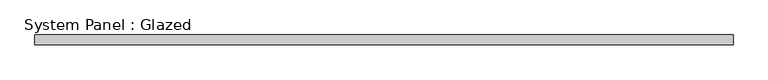
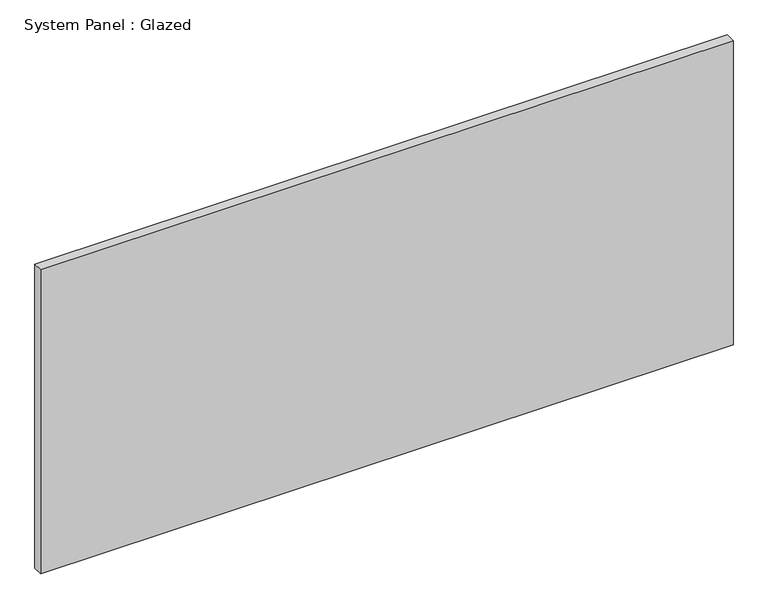
"""IFC4 building model written with IfcOpenShell, lengths in millimetres: plate geometry, System Panel : Glazed."""

import ifcopenshell
import ifcopenshell.guid

model = None  # the IFC model being written
_history = None  # IfcOwnerHistory: only IFC2X3 demands one
_inside = {}  # id of a spatial element -> (the spatial element, [elements in it])
_under = {}  # id of a project, library or spatial element -> (it, [spatial elements below it])
_declared = {}  # id of a project -> (the project, [libraries it declares])
_typed = {}  # id of a type object -> (the type object, [elements of that type])
_made_of = {}  # id of a material, layer set ... -> (it, [elements and type objects made of it])


def new_model(schema):
    """Start an empty IFC model of exactly this schema.

    Asked for "IFC4X3", IfcOpenShell would pick the latest addendum, in which some entities
    have other attributes; the version numbers below select the first issue.
    IFC2X3 requires an IfcOwnerHistory on every rooted entity: one is made here for all.
    """
    global model, _history
    if schema == "IFC4X3":
        model = ifcopenshell.file(schema_version=(4, 3, 0, 0))
    else:
        model = ifcopenshell.file(schema=schema)
    _inside.clear()
    _under.clear()
    _declared.clear()
    _typed.clear()
    _made_of.clear()
    _history = None
    if model.schema == "IFC2X3":
        org = make("IfcOrganization", Name="unknown")
        user = make(
            "IfcPersonAndOrganization",
            ThePerson=make("IfcPerson", FamilyName="unknown"),
            TheOrganization=org,
        )
        app = make(
            "IfcApplication",
            ApplicationDeveloper=org,
            Version="unknown",
            ApplicationFullName="unknown",
            ApplicationIdentifier="unknown",
        )
        _history = make(
            "IfcOwnerHistory",
            OwningUser=user,
            OwningApplication=app,
            ChangeAction="ADDED",
            CreationDate=0,
        )
    return model


def make(cls, **values):
    """One entity of the class cls with the attributes given. An attribute that is None is left unset."""
    return model.create_entity(
        cls, **{name: value for name, value in values.items() if value is not None}
    )


def rooted(cls, **values):
    """An entity with a GlobalId (a new one), such as an element, a storey or a relation."""
    return make(cls, GlobalId=ifcopenshell.guid.new(), OwnerHistory=_history, **values)


def si_unit(unit_type, name, prefix=None):
    """IfcSIUnit, for example si_unit("LENGTHUNIT", "METRE", prefix="MILLI")."""
    return make("IfcSIUnit", UnitType=unit_type, Prefix=prefix, Name=name)


def assignment(units):
    """IfcUnitAssignment: the units of a project."""
    return None if units is None else make("IfcUnitAssignment", Units=units)


def point(xyz):
    """IfcCartesianPoint."""
    return None if xyz is None else make("IfcCartesianPoint", Coordinates=xyz)


def direction(xyz):
    """IfcDirection."""
    return None if xyz is None else make("IfcDirection", DirectionRatios=xyz)


def frame(location, z_axis=None, x_axis=None):
    """IfcAxis2Placement3D, a coordinate frame: its origin and axes. An axis left out is left unset."""
    return make(
        "IfcAxis2Placement3D",
        Location=point(location),
        Axis=direction(z_axis),
        RefDirection=direction(x_axis),
    )


def origin():
    """The frame at (0, 0, 0) with its axes left unset."""
    return frame((0.0, 0.0, 0.0))


def origin_with_axes():
    """The frame at (0, 0, 0) with the z axis (0, 0, 1) and the x axis (1, 0, 0) written out."""
    return frame((0.0, 0.0, 0.0), z_axis=(0.0, 0.0, 1.0), x_axis=(1.0, 0.0, 0.0))


def place(relative_to, where):
    """IfcLocalPlacement: puts the frame where relative to a parent placement (None: the world)."""
    return make(
        "IfcLocalPlacement", PlacementRelTo=relative_to, RelativePlacement=where
    )


def context(
    kind, dimensions, precision=None, world=None, true_north=None, identifier=None
):
    """IfcGeometricRepresentationContext, for example the 3D "Model" context."""
    return make(
        "IfcGeometricRepresentationContext",
        ContextIdentifier=identifier,
        ContextType=kind,
        CoordinateSpaceDimension=dimensions,
        Precision=precision,
        WorldCoordinateSystem=world,
        TrueNorth=true_north,
    )


def project(units=None, contexts=None):
    """IfcProject with its units and contexts."""
    return rooted(
        "IfcProject",
        Name="project",
        RepresentationContexts=contexts,
        UnitsInContext=assignment(units),
    )


def spatial(cls, under=None, at=None, **own):
    """A site, building, storey or space (cls), placed at a placement, below another one or the project."""
    s = rooted(cls, ObjectPlacement=at, **own)
    if under is not None:
        _under.setdefault(under.id(), (under, []))[1].append(s)
    return s


def polyline(points):
    """IfcPolyline through the points."""
    return make("IfcPolyline", Points=[point(p) for p in points])


def outline(outer, holes=None, kind="AREA"):
    """IfcArbitraryClosedProfileDef: a profile drawn as a closed curve; with holes, ...WithVoids."""
    if holes is None:
        return make("IfcArbitraryClosedProfileDef", ProfileType=kind, OuterCurve=outer)
    return make(
        "IfcArbitraryProfileDefWithVoids",
        ProfileType=kind,
        OuterCurve=outer,
        InnerCurves=holes,
    )


def extrude(swept, where, along, depth):
    """IfcExtrudedAreaSolid: the profile swept, set in the frame where, extruded along a direction by depth."""
    return make(
        "IfcExtrudedAreaSolid",
        SweptArea=swept,
        Position=where,
        ExtrudedDirection=direction(along),
        Depth=depth,
    )


def shape(context_of_items, identifier, shape_type, items):
    """IfcShapeRepresentation: the items that make up one representation, for example the "Body"."""
    return make(
        "IfcShapeRepresentation",
        ContextOfItems=context_of_items,
        RepresentationIdentifier=identifier,
        RepresentationType=shape_type,
        Items=items,
    )


def source(mapping_origin, context_of_items, identifier, shape_type, items):
    """IfcRepresentationMap: a shape defined once, which mapped items show again and again."""
    return make(
        "IfcRepresentationMap",
        MappingOrigin=mapping_origin,
        MappedRepresentation=shape(context_of_items, identifier, shape_type, items),
    )


def transform(
    local_origin,
    x_axis=None,
    y_axis=None,
    z_axis=None,
    scale=None,
    scale2=None,
    scale3=None,
    uniform=True,
):
    """IfcCartesianTransformationOperator3D, or its non-uniform kind. x_axis, y_axis, z_axis: its Axis1, 2, 3."""
    if uniform:
        return make(
            "IfcCartesianTransformationOperator3D",
            Axis1=direction(x_axis),
            Axis2=direction(y_axis),
            LocalOrigin=point(local_origin),
            Scale=scale,
            Axis3=direction(z_axis),
        )
    return make(
        "IfcCartesianTransformationOperator3DnonUniform",
        Axis1=direction(x_axis),
        Axis2=direction(y_axis),
        LocalOrigin=point(local_origin),
        Scale=scale,
        Axis3=direction(z_axis),
        Scale2=scale2,
        Scale3=scale3,
    )


def mapped(mapping_source, mapping_target):
    """IfcMappedItem: shows the shape of a source again, moved by a transform."""
    return make(
        "IfcMappedItem", MappingSource=mapping_source, MappingTarget=mapping_target
    )


def made_of(thing, what):
    """Note that an element or type object is made of a material, layer set ...; save() writes the relation."""
    if what is not None:
        _made_of.setdefault(what.id(), (what, []))[1].append(thing)
    return thing


def element(
    cls,
    number,
    at=None,
    inside=None,
    cuts=None,
    type_object=None,
    material=None,
    context=None,
    identifier="Body",
    shape_type=None,
    held_by="IfcProductDefinitionShape",
    body=None,
    shapes=None,
    **own,
):
    """One element of the class cls, such as IfcWall. Its Tag is "e" and its number.

    at: its placement. inside: the storey or other place that contains it. cuts: it is an
    opening in that element (IfcRelVoidsElement). A single representation is given by context,
    identifier, shape_type and body (its items); several are given by shapes. held_by: the class
    of the entity that holds the representations. save() writes the other relations.
    """
    e = rooted(cls, Tag="e%d" % number, ObjectPlacement=at, **own)
    if body is not None:
        shapes = [shape(context, identifier, shape_type, body)]
    if shapes is not None:
        e.Representation = make(held_by, Representations=shapes)
    if inside is not None:
        _inside.setdefault(inside.id(), (inside, []))[1].append(e)
    if cuts is not None:
        rooted(
            "IfcRelVoidsElement", RelatingBuildingElement=cuts, RelatedOpeningElement=e
        )
    if type_object is not None:
        _typed.setdefault(type_object.id(), (type_object, []))[1].append(e)
    return made_of(e, material)


def aggregate(whole, parts):
    """IfcRelAggregates: a whole, such as a stair, and the parts it consists of."""
    return rooted("IfcRelAggregates", RelatingObject=whole, RelatedObjects=parts)


def save(model, path):
    """Write the relations noted so far, then the file.

    IfcRelAggregates (storeys below a building ...), IfcRelContainedInSpatialStructure (elements
    in a storey), IfcRelDefinesByType, IfcRelAssociatesMaterial and IfcRelDeclares: one each for
    every whole, place, type object, material and project.
    """
    for whole, parts in _under.values():
        aggregate(whole, parts)
    for where, things in _inside.values():
        rooted(
            "IfcRelContainedInSpatialStructure",
            RelatedElements=things,
            RelatingStructure=where,
        )
    for kind, things in _typed.values():
        rooted("IfcRelDefinesByType", RelatedObjects=things, RelatingType=kind)
    for what, things in _made_of.values():
        rooted("IfcRelAssociatesMaterial", RelatedObjects=things, RelatingMaterial=what)
    for by, libraries in _declared.values():
        rooted("IfcRelDeclares", RelatingContext=by, RelatedDefinitions=libraries)
    model.write(path)


def system_panel_glazed_f11ab94e(model_context):
    return source(origin(), model_context, "Body", "SweptSolid", [
        extrude(outline(polyline([(882.65, -44.45), (-882.65, -44.45), (-882.65, -19.05), (882.65, -19.05), (882.65, -44.45)])), origin_with_axes(), (0.0, 0.0, 1.0), 819.15),
    ])


if __name__ == "__main__":
    model = new_model("IFC4")
    model_context = context("Model", 3, world=origin())
    ifc_project = project(units=[si_unit("LENGTHUNIT", "METRE", prefix="MILLI")], contexts=[model_context])
    site = spatial("IfcSite", under=ifc_project)
    building = spatial("IfcBuilding", under=site)
    placement = place(None, origin())
    system_panel_glazed_shape = system_panel_glazed_f11ab94e(model_context)
    element("IfcPlate", 1, ObjectType="System Panel : Glazed", at=placement, inside=building, context=model_context, shape_type="MappedRepresentation", body=[
        mapped(system_panel_glazed_shape, transform((0.0, 0.0, 0.0), x_axis=(1.0, 0.0, 0.0), y_axis=(0.0, 1.0, 0.0), z_axis=(0.0, 0.0, 1.0))),
    ])
    save(model, "model.ifc")

# Revit data of these elements
# Type "System Panel : Glazed"
#   Construction Type Id = "GSP4R"
#   Analytic Construction = "1/8 in Pilkington single glazing"
#   Visual Light Transmittance = 0.9
#   Solar Heat Gain Coefficient = 0.86
#   Heat Transfer Coefficient (U) = 1.18115 BTU/(h·ft²·°F)
#   Define Thermal Properties by = 1
# Element 1 (IfcPlate, "System Panel : Glazed")
#   Materials on its faces: "Glass"
# Materials
#   "Glass": class "Glass", colour RGB 0 128 192, transparency 0.75, Description = "Soda Lime Glass", Cost = 0
